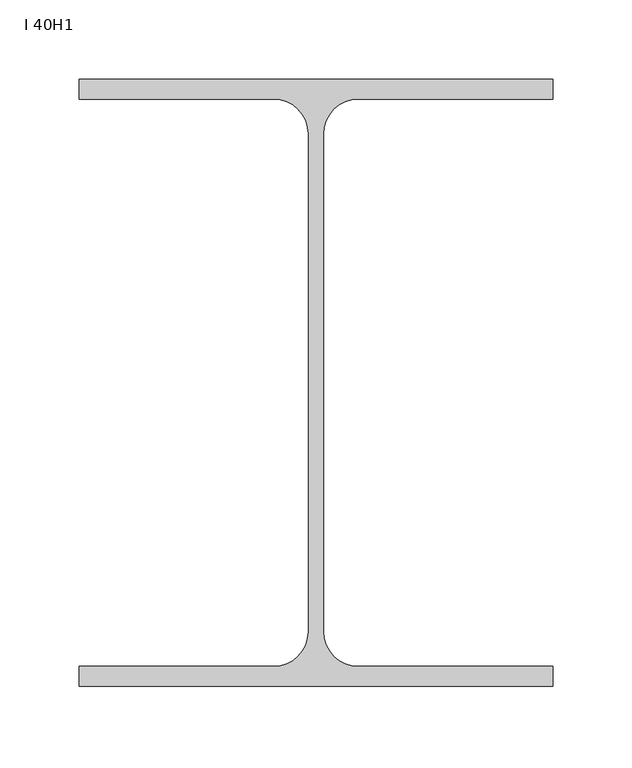
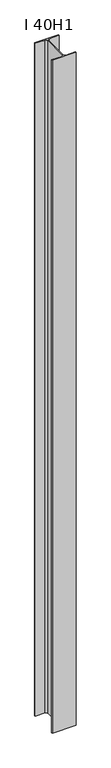
"""IFC4 building model written with IfcOpenShell, lengths in millimetres: column geometry, Двутавровая балка с широкими полками (ASTO20-93)-Колонна : I 40H1."""

from ifc_helpers import new_model, si_unit, point, frame_2d, origin, origin_with_axes, place, context, project, spatial, polyline, circle_curve, trimmed, segment, composite_curve, outline, extrude, source, transform, mapped, element, save


def i_40h1_0f399548(model_context):
    return source(origin(), model_context, "Body", "SweptSolid", [
        extrude(outline(composite_curve([segment(polyline([(-149.5, 178.5), (-149.5, 191.0), (149.5, 191.0), (149.5, 178.5), (26.75, 178.5)]), True, "CONTINUOUS"), segment(trimmed(circle_curve(frame_2d((26.75, 156.5)), 22.0), [point((26.75, 178.5))], [point((4.75, 156.5))], True, "CARTESIAN"), True, "CONTINUOUS"), segment(polyline([(4.75, 156.5), (4.75, -157.5)]), True, "CONTINUOUS"), segment(trimmed(circle_curve(frame_2d((26.75, -157.5)), 22.0), [point((4.75, -157.5))], [point((26.75, -179.5))], True, "CARTESIAN"), True, "CONTINUOUS"), segment(polyline([(26.75, -179.5), (149.5, -179.5), (149.5, -192.0), (-149.5, -192.0), (-149.5, -179.5), (-26.75, -179.5)]), True, "CONTINUOUS"), segment(trimmed(circle_curve(frame_2d((-26.75, -157.5)), 22.0), [point((-26.75, -179.5))], [point((-4.75, -157.5))], True, "CARTESIAN"), True, "CONTINUOUS"), segment(polyline([(-4.75, -157.5), (-4.75, 156.5)]), True, "CONTINUOUS"), segment(trimmed(circle_curve(frame_2d((-26.75, 156.5)), 22.0), [point((-4.75, 156.5))], [point((-26.75, 178.5))], True, "CARTESIAN"), True, "CONTINUOUS"), segment(polyline([(-26.75, 178.5), (-149.5, 178.5)]), True, "CONTINUOUS")], self_intersect=False)), origin_with_axes(), (0.0, 0.0, 1.0), 8923.3858447),
    ])


if __name__ == "__main__":
    model = new_model("IFC4")
    model_context = context("Model", 3, world=origin())
    ifc_project = project(units=[si_unit("LENGTHUNIT", "METRE", prefix="MILLI")], contexts=[model_context])
    site = spatial("IfcSite", under=ifc_project)
    building = spatial("IfcBuilding", under=site)
    placement = place(None, origin())
    i_40h1_shape = i_40h1_0f399548(model_context)
    element("IfcColumn", 1, ObjectType="Двутавровая балка с широкими полками (ASTO20-93)-Колонна : I 40H1", at=placement, inside=building, context=model_context, shape_type="MappedRepresentation", body=[
        mapped(i_40h1_shape, transform((0.0, 0.0, 0.0), x_axis=(1.0, 0.0, 0.0), y_axis=(0.0, 1.0, 0.0), z_axis=(0.0, 0.0, 1.0))),
    ])
    save(model, "model.ifc")

# Revit data of these elements
# Type "Двутавровая балка с широкими полками (ASTO20-93)-Колонна : I 40H1"
#   ra = 22 mm
#   W = 0.868869
#   Vz = 191.5 mm
#   Vy = 149.5 mm
#   Vpz = 191.5 mm
#   Vpy = 149.5 mm
#   bf = 299 mm
#   d = 383 mm
#   tf = 12.5 mm
#   tw = 9.5 mm
#   A = 0.011291 m²
#   Structural Material [instance default] = Металл - Сталь - 345 МПa
#   Assembly Code = ""
# Element 1 (IfcColumn, "Двутавровая балка с широкими полками (ASTO20-93)-Колонна : I 40H1")
#   Structural Material = C345
#   Materials on its faces: "C345"
# Materials
#   "Металл - Сталь - 345 МПa": class "Металл", colour RGB 247 247 247, transparency 0
#   "C345": class "Не назначено", colour RGB 0 0 0, transparency 0
